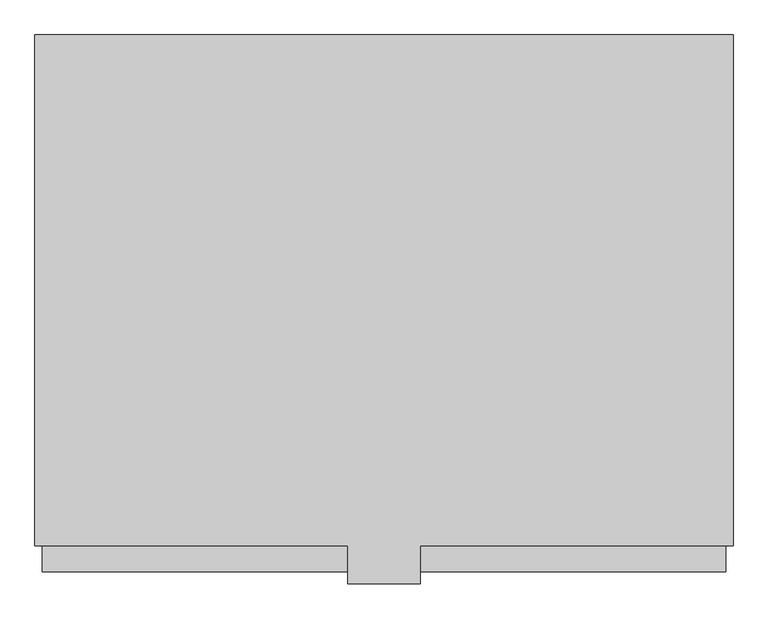
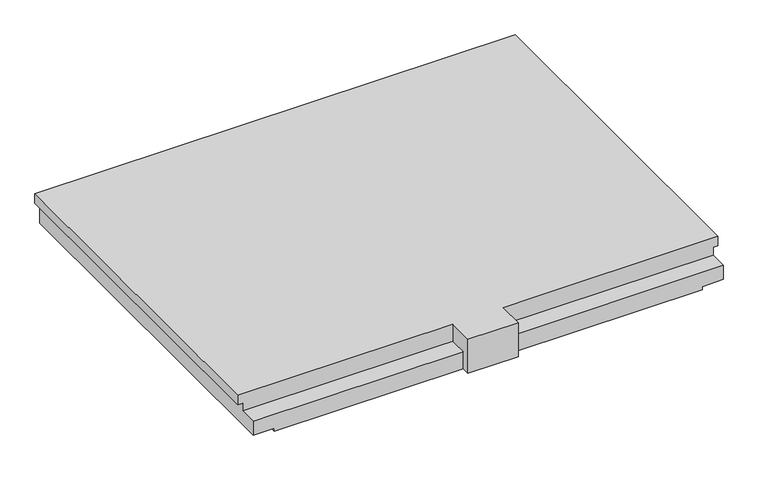
"""IFC4 building model written with IfcOpenShell, lengths in millimetres: proxy geometry, NLRS_24_GM_UN_rechthoekig bordes prefab-AV_gen_rsf : prefab bordes_gen__2250x2925."""

from ifc_helpers import new_model, si_unit, origin, place, context, project, spatial, faceted_brep, source, transform, mapped, element, save


def generic_models_ecb21330(model_context):
    return source(origin(), model_context, "Body", "Brep", [
        faceted_brep([(1462.5, -2140.0, 0.0), (1462.5, -2140.0, -60.0), (1462.5, 0.0, -60.0), (1462.5, 0.0, 0.0), (152.5, -2250.0, -110.0), (1432.5, -2250.0, -110.0), (1432.5, -2140.0, -110.0), (152.5, -2140.0, -110.0), (152.5, -2140.0, 0.0), (1432.5, -2140.0, -60.0), (152.5, -2300.0, -220.0), (152.5, -2250.0, -220.0), (152.5, -2300.0, 0.0), (-152.5, -2300.0, 0.0), (-152.5, -2140.0, 0.0), (-152.5, -2140.0, -110.0), (-152.5, -2250.0, -110.0), (-152.5, -2250.0, -220.0), (-152.5, -2300.0, -220.0), (-1462.5, 0.0, 0.0), (-1462.5, 0.0, -60.0), (-1462.5, -2140.0, -60.0), (-1462.5, -2140.0, 0.0), (-1432.5, -2250.0, -110.0), (-1432.5, -2250.0, -200.0), (-1302.5, -2250.0, -200.0), (-1302.5, -2250.0, -220.0), (-1432.5, -2140.0, -110.0), (-1432.5, -2140.0, -60.0), (1432.5, 0.0, -60.0), (1432.5, 0.0, -200.0), (1302.5, 0.0, -200.0), (1302.5, 0.0, -220.0), (-1302.5, 0.0, -220.0), (-1302.5, 0.0, -200.0), (-1432.5, 0.0, -200.0), (-1432.5, 0.0, -60.0), (1302.5, -2250.0, -220.0), (1432.5, -2250.0, -200.0), (1302.5, -2250.0, -200.0)], [[[0, 1, 2, 3]], [[4, 5, 6, 7]], [[8, 7, 6, 9, 1, 0]], [[10, 11, 4, 7, 8, 12]], [[13, 14, 15, 16, 17, 18]], [[19, 20, 21, 22]], [[17, 16, 23, 24, 25, 26]], [[16, 15, 27, 23]], [[22, 21, 28, 27, 15, 14]], [[22, 14, 13, 12, 8, 0, 3, 19]], [[19, 3, 2, 29, 30, 31, 32, 33, 34, 35, 36, 20]], [[26, 33, 32, 37, 11, 10, 18, 17]], [[28, 21, 20, 36]], [[24, 23, 27, 28, 36, 35]], [[35, 34, 25, 24]], [[34, 33, 26, 25]], [[29, 2, 1, 9]], [[9, 6, 5, 38, 30, 29]], [[38, 39, 31, 30]], [[39, 37, 32, 31]], [[11, 37, 39, 38, 5, 4]], [[12, 13, 18, 10]]]),
    ])


if __name__ == "__main__":
    model = new_model("IFC4")
    model_context = context("Model", 3, world=origin())
    ifc_project = project(units=[si_unit("LENGTHUNIT", "METRE", prefix="MILLI")], contexts=[model_context])
    site = spatial("IfcSite", under=ifc_project)
    building = spatial("IfcBuilding", under=site)
    placement = place(None, origin())
    generic_models_shape = generic_models_ecb21330(model_context)
    element("IfcBuildingElementProxy", 1, Name="NLRS_24_GM_UN_rechthoekig bordes prefab-AV_gen_rsf : prefab bordes_gen__2250x2925", ObjectType="NLRS_24_GM_UN_rechthoekig bordes prefab-AV_gen_rsf : prefab bordes_gen__2250x2925", at=placement, inside=building, context=model_context, shape_type="MappedRepresentation", body=[
        mapped(generic_models_shape, transform((0.0, 0.0, 0.0), x_axis=(1.0, 0.0, 0.0), y_axis=(0.0, 1.0, 0.0), z_axis=(0.0, 0.0, 1.0))),
    ])
    save(model, "model.ifc")

# Revit data of these elements
# Type "NLRS_24_GM_UN_rechthoekig bordes prefab-AV_gen_rsf : prefab bordes_gen__2250x2925"
#   Export Type to IFC As = "IfcStair"
#   Type IfcGUID = "2CEqVLPNH8KRN7ghwV3bMM"
#   Type Comments = " "
#   Model = " "
#   Manufacturer = " "
#   Description = "rechthoekig bordes prefab\r\n1930x4395"
#   Assembly Code = "24.15"
#   Width = 2925 mm
#   Thickness = 220 mm
#   Perimeter = 10450 mm
#   NLRS_C_lengte_02 = 1310 mm
#   NLRS_C_lengte_01 = 1310 mm
#   NLRS_C_hoogte_02 = 110 mm
#   NLRS_C_hoogte_01 = 110 mm
#   NLRS_C_diepte_04 = 2250 mm
#   NLRS_C_diepte_03 = 2250 mm
#   NLRS_C_diepte_02 = 110 mm
#   NLRS_C_diepte_01 = 110 mm
#   Length = 2300 mm
#   Default Elevation = 1219.2 mm
#   Area = 6.7275 m²
#   NLRS_C_materiaal = NLRS_f2_beton prefab_gen_rsf
#   Keynote = ""
# Element 1 (IfcBuildingElementProxy, "NLRS_24_GM_UN_rechthoekig bordes prefab-AV_gen_rsf : prefab bordes_gen__2250x2925")
#   Materials on its faces: "NLRS_f2_beton prefab_gen_rsf"
# Materials
#   "NLRS_f2_beton prefab_gen_rsf": class "F - Niet gebakken kunststeen", colour RGB 129 133 118, transparency 0, Keynote = "f2", Manufacturer = "Revit Standards Foundation", URL = "www.revitstandards.org", Description = "beton prefab", Cost = 0
